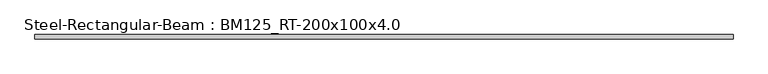
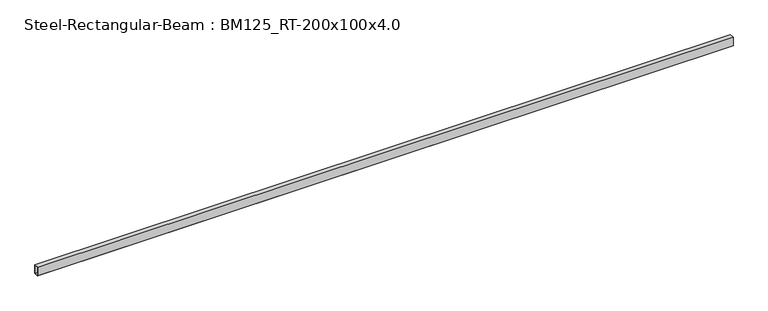
"""IFC4 building model written with IfcOpenShell, lengths in millimetres: beam geometry, Steel-Rectangular-Beam : BM125_RT-200x100x4.0."""

from ifc_helpers import new_model, si_unit, frame, origin, place, context, project, spatial, polyline, outline, extrude, source, transform, mapped, element, save


def steel_rectangular_beam_bm125_rt_200x100x4_0_de2c2afd(model_context):
    return source(origin(), model_context, "Body", "SweptSolid", [
        extrude(outline(polyline([(50.0, 100.0), (50.0, -100.0), (-50.0, -100.0), (-50.0, 100.0), (50.0, 100.0)]), holes=[polyline([(-46.0, -96.0), (46.0, -96.0), (46.0, 96.0), (-46.0, 96.0), (-46.0, -96.0)])]), frame((-7500.0, 0.0, 0.0), z_axis=(1.0, 0.0, 0.0), x_axis=(0.0, 1.0, 0.0)), (0.0, 0.0, 1.0), 15500.0),
        extrude(outline(polyline([(50.0, 100.0), (50.0, -100.0), (-50.0, -100.0), (-50.0, 100.0), (50.0, 100.0)]), holes=[polyline([(-46.0, -96.0), (46.0, -96.0), (46.0, 96.0), (-46.0, 96.0), (-46.0, -96.0)])]), frame((-7500.0, 0.0, 0.0), z_axis=(1.0, 0.0, 0.0), x_axis=(0.0, 1.0, 0.0)), (0.0, 0.0, 1.0), 15500.0),
        extrude(outline(polyline([(50.0, 100.0), (50.0, -100.0), (-50.0, -100.0), (-50.0, 100.0), (50.0, 100.0)]), holes=[polyline([(-46.0, -96.0), (46.0, -96.0), (46.0, 96.0), (-46.0, 96.0), (-46.0, -96.0)])]), frame((-7500.0, 0.0, 0.0), z_axis=(1.0, 0.0, 0.0), x_axis=(0.0, 1.0, 0.0)), (0.0, 0.0, 1.0), 15500.0),
        extrude(outline(polyline([(50.0, 100.0), (50.0, -100.0), (-50.0, -100.0), (-50.0, 100.0), (50.0, 100.0)]), holes=[polyline([(-46.0, -96.0), (46.0, -96.0), (46.0, 96.0), (-46.0, 96.0), (-46.0, -96.0)])]), frame((-7500.0, 0.0, 0.0), z_axis=(1.0, 0.0, 0.0), x_axis=(0.0, 1.0, 0.0)), (0.0, 0.0, 1.0), 15500.0),
    ])


if __name__ == "__main__":
    model = new_model("IFC4")
    model_context = context("Model", 3, world=origin())
    ifc_project = project(units=[si_unit("LENGTHUNIT", "METRE", prefix="MILLI")], contexts=[model_context])
    site = spatial("IfcSite", under=ifc_project)
    building = spatial("IfcBuilding", under=site)
    placement = place(None, origin())
    steel_rectangular_beam_bm125_rt_200x100x4_0_shape = steel_rectangular_beam_bm125_rt_200x100x4_0_de2c2afd(model_context)
    element("IfcBeam", 1, ObjectType="Steel-Rectangular-Beam : BM125_RT-200x100x4.0", at=placement, inside=building, context=model_context, shape_type="MappedRepresentation", body=[
        mapped(steel_rectangular_beam_bm125_rt_200x100x4_0_shape, transform((0.0, 0.0, 0.0), x_axis=(1.0, 0.0, 0.0), y_axis=(0.0, 1.0, 0.0), z_axis=(0.0, 0.0, 1.0))),
    ])
    save(model, "model.ifc")

# Revit data of these elements
# Type "Steel-Rectangular-Beam : BM125_RT-200x100x4.0"
#   t = 4 mm
#   Mass per Unit Length = 18.35 kg/m
#   Surface Area = 0.60 m²/m
#   Sectional Area = 1856.0 cm²
#   Length [instance default] = 3000 mm
#   H = 200 mm
#   B = 100 mm
#   hec_material4 [instance default] = none
#   hec_material3 [instance default] = none
#   hec_material2 [instance default] = none
#   hec_material1 [instance default] = none
#   Structural Material [instance default] = none
# Element 1 (IfcBeam, "Steel-Rectangular-Beam : BM125_RT-200x100x4.0")
#   hec_material2 = S01AA010-00001_Main Steel Structure Fabrication Work_Shelter/Building_Steel Painting/Coating_for Non-Fireproofed Steel Surface, Surface Preparation, Primer, Second & Final Coat
#   hec_material1 = S03AA007-00001_Main Steel Structure Erection Work_Girth & Purlin
#   Structural Material = S01AA007-00001_Main Steel Structure Fabrication Work_Shelter/Building_Girth & Purlin
#   Materials on its faces: "S01AA010-00001_Main Steel Structure Fabrication Work_Shelter/Building_Steel Painting/Coating_for Non-Fireproofed Steel Surface, Surface Preparation, Primer, Second & Final Coat"
# Materials
#   "S01AA010-00001_Main Steel Structure Fabrication Work_Shelter/Building_Steel Painting/Coating_for Non-Fireproofed Steel Surface, Surface Preparation, Primer, Second & Final Coat": class "Metal", colour RGB 120 120 120, transparency 0, Description = "Paint finished steel", W00) Work Master Code = "S01AA010-00001", W01) Work Master_Lv1 = "Main Steel Structure Fabrication Work", W02) Work Master_Lv2 = "Shelter/Building", W03) Work Master_Spec.1 = "Steel Painting/Coating", W04) Work Master_Spec.2 = "for Non-Fireproofed Steel Surface, Surface Preparation, Primer, Second & Final Coat", Cost = 0
#   "S03AA007-00001_Main Steel Structure Erection Work_Girth & Purlin": class "Metal", colour RGB 120 120 120, transparency 0, Comments = "(30KG/M>Weight)", Description = "Structural steel 50ksi", W00) Work Master Code = "S03AA007-00001", W01) Work Master_Lv1 = "Main Steel Structure Erection Work", W02) Work Master_Lv2 = "Shelter/Building", W03) Work Master_Spec.1 = "Girth & Purlin", Cost = 0
#   "S01AA007-00001_Main Steel Structure Fabrication Work_Shelter/Building_Girth & Purlin": class "Metal", colour RGB 120 120 120, transparency 0, Comments = "(30KG/M>Weight)", Description = "Structural steel 50ksi", W00) Work Master Code = "S01AA007-00001", W01) Work Master_Lv1 = "Main Steel Structure Fabrication Work", W02) Work Master_Lv2 = "Shelter/Building", W03) Work Master_Spec.1 = "Girth & Purlin", Cost = 0
